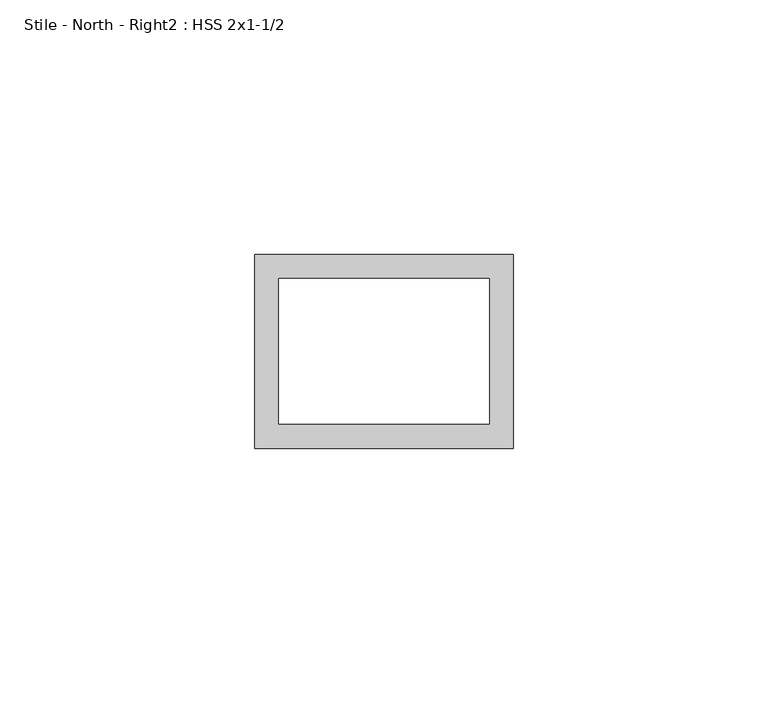
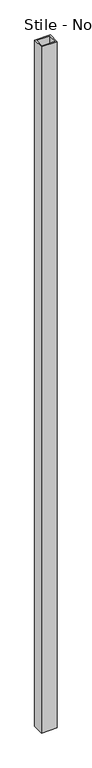
"""IFC4 building model written with IfcOpenShell, lengths in millimetres: proxy geometry, Stile - North - Right2 : HSS 2x1-1/2."""

from ifc_helpers import new_model, si_unit, frame, origin, place, context, project, spatial, polyline, outline, extrude, source, transform, mapped, element, save


def stile_north_right2_hss_2x1_1_2_44639784(model_context):
    return source(origin(), model_context, "Body", "SweptSolid", [
        extrude(outline(polyline([(587365.8934739, -532839.3663841), (587416.6934739, -532839.3663841), (587416.6934739, -532877.4663841), (587365.8934739, -532877.4663841), (587365.8934739, -532839.3663841)]), holes=[polyline([(587370.6559739, -532844.1288841), (587370.6559739, -532872.7038841), (587411.9309739, -532872.7038841), (587411.9309739, -532844.1288841), (587370.6559739, -532844.1288841)])]), frame((0.0, 0.0, 50.8), z_axis=(0.0, 0.0, 1.0), x_axis=(1.0, 0.0, 0.0)), (0.0, 0.0, 1.0), 2349.5),
    ])


if __name__ == "__main__":
    model = new_model("IFC4")
    model_context = context("Model", 3, world=origin())
    ifc_project = project(units=[si_unit("LENGTHUNIT", "METRE", prefix="MILLI")], contexts=[model_context])
    site = spatial("IfcSite", under=ifc_project)
    building = spatial("IfcBuilding", under=site)
    placement = place(None, origin())
    stile_north_right2_hss_2x1_1_2_shape = stile_north_right2_hss_2x1_1_2_44639784(model_context)
    element("IfcBuildingElementProxy", 1, Name="Stile - North - Right2 : HSS 2x1-1/2", ObjectType="Stile - North - Right2 : HSS 2x1-1/2", at=placement, inside=building, context=model_context, shape_type="MappedRepresentation", body=[
        mapped(stile_north_right2_hss_2x1_1_2_shape, transform((0.0, 0.0, 0.0), x_axis=(1.0, 0.0, 0.0), y_axis=(0.0, 1.0, 0.0), z_axis=(0.0, 0.0, 1.0))),
    ])
    save(model, "model.ifc")

# Revit data of these elements
# Element 1 (IfcBuildingElementProxy, "Stile - North - Right2 : HSS 2x1-1/2")
#   Materials on its faces: "1-1/2\"X2\" GALV. STL HSS TUBING"
# Materials
#   "1-1/2\"X2\" GALV. STL HSS TUBING": class "Generic", colour RGB 211 211 207, transparency 0, Cost = 0
